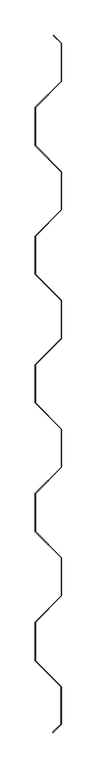
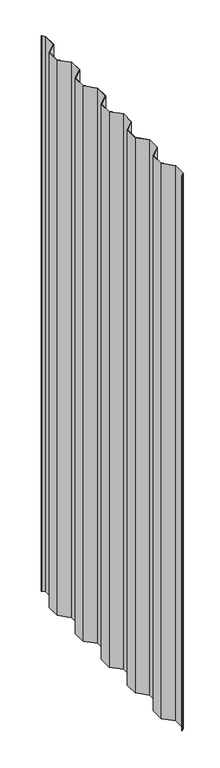
"""IFC4 building model written with IfcOpenShell, lengths in millimetres: proxy geometry, MBCI 7.2-V Panel22 : MBCI 7.2-V Panel-1."""

import ifcopenshell
import ifcopenshell.guid

model = None  # the IFC model being written
_history = None  # IfcOwnerHistory: only IFC2X3 demands one
_inside = {}  # id of a spatial element -> (the spatial element, [elements in it])
_under = {}  # id of a project, library or spatial element -> (it, [spatial elements below it])
_declared = {}  # id of a project -> (the project, [libraries it declares])
_typed = {}  # id of a type object -> (the type object, [elements of that type])
_made_of = {}  # id of a material, layer set ... -> (it, [elements and type objects made of it])


def new_model(schema):
    """Start an empty IFC model of exactly this schema.

    Asked for "IFC4X3", IfcOpenShell would pick the latest addendum, in which some entities
    have other attributes; the version numbers below select the first issue.
    IFC2X3 requires an IfcOwnerHistory on every rooted entity: one is made here for all.
    """
    global model, _history
    if schema == "IFC4X3":
        model = ifcopenshell.file(schema_version=(4, 3, 0, 0))
    else:
        model = ifcopenshell.file(schema=schema)
    _inside.clear()
    _under.clear()
    _declared.clear()
    _typed.clear()
    _made_of.clear()
    _history = None
    if model.schema == "IFC2X3":
        org = make("IfcOrganization", Name="unknown")
        user = make(
            "IfcPersonAndOrganization",
            ThePerson=make("IfcPerson", FamilyName="unknown"),
            TheOrganization=org,
        )
        app = make(
            "IfcApplication",
            ApplicationDeveloper=org,
            Version="unknown",
            ApplicationFullName="unknown",
            ApplicationIdentifier="unknown",
        )
        _history = make(
            "IfcOwnerHistory",
            OwningUser=user,
            OwningApplication=app,
            ChangeAction="ADDED",
            CreationDate=0,
        )
    return model


def make(cls, **values):
    """One entity of the class cls with the attributes given. An attribute that is None is left unset."""
    return model.create_entity(
        cls, **{name: value for name, value in values.items() if value is not None}
    )


def rooted(cls, **values):
    """An entity with a GlobalId (a new one), such as an element, a storey or a relation."""
    return make(cls, GlobalId=ifcopenshell.guid.new(), OwnerHistory=_history, **values)


def si_unit(unit_type, name, prefix=None):
    """IfcSIUnit, for example si_unit("LENGTHUNIT", "METRE", prefix="MILLI")."""
    return make("IfcSIUnit", UnitType=unit_type, Prefix=prefix, Name=name)


def assignment(units):
    """IfcUnitAssignment: the units of a project."""
    return None if units is None else make("IfcUnitAssignment", Units=units)


def point(xyz):
    """IfcCartesianPoint."""
    return None if xyz is None else make("IfcCartesianPoint", Coordinates=xyz)


def direction(xyz):
    """IfcDirection."""
    return None if xyz is None else make("IfcDirection", DirectionRatios=xyz)


def frame(location, z_axis=None, x_axis=None):
    """IfcAxis2Placement3D, a coordinate frame: its origin and axes. An axis left out is left unset."""
    return make(
        "IfcAxis2Placement3D",
        Location=point(location),
        Axis=direction(z_axis),
        RefDirection=direction(x_axis),
    )


def origin():
    """The frame at (0, 0, 0) with its axes left unset."""
    return frame((0.0, 0.0, 0.0))


def place(relative_to, where):
    """IfcLocalPlacement: puts the frame where relative to a parent placement (None: the world)."""
    return make(
        "IfcLocalPlacement", PlacementRelTo=relative_to, RelativePlacement=where
    )


def context(
    kind, dimensions, precision=None, world=None, true_north=None, identifier=None
):
    """IfcGeometricRepresentationContext, for example the 3D "Model" context."""
    return make(
        "IfcGeometricRepresentationContext",
        ContextIdentifier=identifier,
        ContextType=kind,
        CoordinateSpaceDimension=dimensions,
        Precision=precision,
        WorldCoordinateSystem=world,
        TrueNorth=true_north,
    )


def project(units=None, contexts=None):
    """IfcProject with its units and contexts."""
    return rooted(
        "IfcProject",
        Name="project",
        RepresentationContexts=contexts,
        UnitsInContext=assignment(units),
    )


def spatial(cls, under=None, at=None, **own):
    """A site, building, storey or space (cls), placed at a placement, below another one or the project."""
    s = rooted(cls, ObjectPlacement=at, **own)
    if under is not None:
        _under.setdefault(under.id(), (under, []))[1].append(s)
    return s


def polyline(points):
    """IfcPolyline through the points."""
    return make("IfcPolyline", Points=[point(p) for p in points])


def outline(outer, holes=None, kind="AREA"):
    """IfcArbitraryClosedProfileDef: a profile drawn as a closed curve; with holes, ...WithVoids."""
    if holes is None:
        return make("IfcArbitraryClosedProfileDef", ProfileType=kind, OuterCurve=outer)
    return make(
        "IfcArbitraryProfileDefWithVoids",
        ProfileType=kind,
        OuterCurve=outer,
        InnerCurves=holes,
    )


def extrude(swept, where, along, depth):
    """IfcExtrudedAreaSolid: the profile swept, set in the frame where, extruded along a direction by depth."""
    return make(
        "IfcExtrudedAreaSolid",
        SweptArea=swept,
        Position=where,
        ExtrudedDirection=direction(along),
        Depth=depth,
    )


def shape(context_of_items, identifier, shape_type, items):
    """IfcShapeRepresentation: the items that make up one representation, for example the "Body"."""
    return make(
        "IfcShapeRepresentation",
        ContextOfItems=context_of_items,
        RepresentationIdentifier=identifier,
        RepresentationType=shape_type,
        Items=items,
    )


def source(mapping_origin, context_of_items, identifier, shape_type, items):
    """IfcRepresentationMap: a shape defined once, which mapped items show again and again."""
    return make(
        "IfcRepresentationMap",
        MappingOrigin=mapping_origin,
        MappedRepresentation=shape(context_of_items, identifier, shape_type, items),
    )


def transform(
    local_origin,
    x_axis=None,
    y_axis=None,
    z_axis=None,
    scale=None,
    scale2=None,
    scale3=None,
    uniform=True,
):
    """IfcCartesianTransformationOperator3D, or its non-uniform kind. x_axis, y_axis, z_axis: its Axis1, 2, 3."""
    if uniform:
        return make(
            "IfcCartesianTransformationOperator3D",
            Axis1=direction(x_axis),
            Axis2=direction(y_axis),
            LocalOrigin=point(local_origin),
            Scale=scale,
            Axis3=direction(z_axis),
        )
    return make(
        "IfcCartesianTransformationOperator3DnonUniform",
        Axis1=direction(x_axis),
        Axis2=direction(y_axis),
        LocalOrigin=point(local_origin),
        Scale=scale,
        Axis3=direction(z_axis),
        Scale2=scale2,
        Scale3=scale3,
    )


def mapped(mapping_source, mapping_target):
    """IfcMappedItem: shows the shape of a source again, moved by a transform."""
    return make(
        "IfcMappedItem", MappingSource=mapping_source, MappingTarget=mapping_target
    )


def made_of(thing, what):
    """Note that an element or type object is made of a material, layer set ...; save() writes the relation."""
    if what is not None:
        _made_of.setdefault(what.id(), (what, []))[1].append(thing)
    return thing


def element(
    cls,
    number,
    at=None,
    inside=None,
    cuts=None,
    type_object=None,
    material=None,
    context=None,
    identifier="Body",
    shape_type=None,
    held_by="IfcProductDefinitionShape",
    body=None,
    shapes=None,
    **own,
):
    """One element of the class cls, such as IfcWall. Its Tag is "e" and its number.

    at: its placement. inside: the storey or other place that contains it. cuts: it is an
    opening in that element (IfcRelVoidsElement). A single representation is given by context,
    identifier, shape_type and body (its items); several are given by shapes. held_by: the class
    of the entity that holds the representations. save() writes the other relations.
    """
    e = rooted(cls, Tag="e%d" % number, ObjectPlacement=at, **own)
    if body is not None:
        shapes = [shape(context, identifier, shape_type, body)]
    if shapes is not None:
        e.Representation = make(held_by, Representations=shapes)
    if inside is not None:
        _inside.setdefault(inside.id(), (inside, []))[1].append(e)
    if cuts is not None:
        rooted(
            "IfcRelVoidsElement", RelatingBuildingElement=cuts, RelatedOpeningElement=e
        )
    if type_object is not None:
        _typed.setdefault(type_object.id(), (type_object, []))[1].append(e)
    return made_of(e, material)


def aggregate(whole, parts):
    """IfcRelAggregates: a whole, such as a stair, and the parts it consists of."""
    return rooted("IfcRelAggregates", RelatingObject=whole, RelatedObjects=parts)


def save(model, path):
    """Write the relations noted so far, then the file.

    IfcRelAggregates (storeys below a building ...), IfcRelContainedInSpatialStructure (elements
    in a storey), IfcRelDefinesByType, IfcRelAssociatesMaterial and IfcRelDeclares: one each for
    every whole, place, type object, material and project.
    """
    for whole, parts in _under.values():
        aggregate(whole, parts)
    for where, things in _inside.values():
        rooted(
            "IfcRelContainedInSpatialStructure",
            RelatedElements=things,
            RelatingStructure=where,
        )
    for kind, things in _typed.values():
        rooted("IfcRelDefinesByType", RelatedObjects=things, RelatingType=kind)
    for what, things in _made_of.values():
        rooted("IfcRelAssociatesMaterial", RelatedObjects=things, RelatingMaterial=what)
    for by, libraries in _declared.values():
        rooted("IfcRelDeclares", RelatingContext=by, RelatedDefinitions=libraries)
    model.write(path)


def generic_models_8da91ac8(model_context):
    return source(origin(), model_context, "Body", "SweptSolid", [
        extrude(outline(polyline([(587368.2461489, -533059.7470706), (587330.7557489, -533097.2374706), (587330.7557489, -533151.0249614), (587368.2461489, -533188.5153614), (587368.2461489, -533242.6270706), (587330.7557489, -533280.1174706), (587330.7557489, -533333.9049614), (587368.2461489, -533371.3953614), (587368.2461489, -533425.5070706), (587330.7557489, -533462.9974706), (587330.7557489, -533516.7849614), (587368.2461489, -533554.2753614), (587368.2461489, -533608.3870706), (587330.7557489, -533645.8774706), (587330.7557489, -533699.6649614), (587368.2461489, -533737.1553614), (587368.2461489, -533791.2670706), (587330.7557489, -533828.7574706), (587330.7557489, -533883.4085614), (587367.6365489, -533920.2893614), (587367.6365489, -533973.8706614), (587355.9658262, -533985.5413841), (587355.9108025, -533984.7545088), (587367.0412364, -533973.6240749), (587367.0412364, -533920.5359479), (587330.1604364, -533883.6551479), (587330.1604364, -533828.510884), (587367.6508364, -533791.020484), (587367.6508364, -533737.4019479), (587330.1604364, -533699.9115479), (587330.1604364, -533645.630884), (587367.6508364, -533608.140484), (587367.6508364, -533554.5219479), (587330.1604364, -533517.0315479), (587330.1604364, -533462.750884), (587367.6508364, -533425.260484), (587367.6508364, -533371.6419479), (587330.1604364, -533334.1515479), (587330.1604364, -533279.870884), (587367.6508364, -533242.380484), (587367.6508364, -533188.7619479), (587330.1604364, -533151.2715479), (587330.1604364, -533096.990884), (587367.6508364, -533059.500484), (587367.6508364, -533005.8819479), (587356.8035899, -532995.0347014), (587356.8455148, -532994.2347273), (587368.2461489, -533005.6353614), (587368.2461489, -533059.7470706)])), frame((0.0, 0.0, 51.59375), z_axis=(0.0, 0.0, 1.0), x_axis=(1.0, 0.0, 0.0)), (0.0, 0.0, 1.0), 2386.80625),
    ])


if __name__ == "__main__":
    model = new_model("IFC4")
    model_context = context("Model", 3, world=origin())
    ifc_project = project(units=[si_unit("LENGTHUNIT", "METRE", prefix="MILLI")], contexts=[model_context])
    site = spatial("IfcSite", under=ifc_project)
    building = spatial("IfcBuilding", under=site)
    placement = place(None, origin())
    generic_models_shape = generic_models_8da91ac8(model_context)
    element("IfcBuildingElementProxy", 1, Name="MBCI 7.2-V Panel22 : MBCI 7.2-V Panel-1", ObjectType="MBCI 7.2-V Panel22 : MBCI 7.2-V Panel-1", at=placement, inside=building, context=model_context, shape_type="MappedRepresentation", body=[
        mapped(generic_models_shape, transform((0.0, 0.0, 0.0), x_axis=(1.0, 0.0, 0.0), y_axis=(0.0, 1.0, 0.0), z_axis=(0.0, 0.0, 1.0))),
    ])
    save(model, "model.ifc")

# Revit data of these elements
# Element 1 (IfcBuildingElementProxy, "MBCI 7.2-V Panel22 : MBCI 7.2-V Panel-1")
#   Materials on its faces: "MTL PANEL"
# Materials
#   "MTL PANEL": class "Generic", colour RGB 239 242 240, transparency 0, Cost = 0
